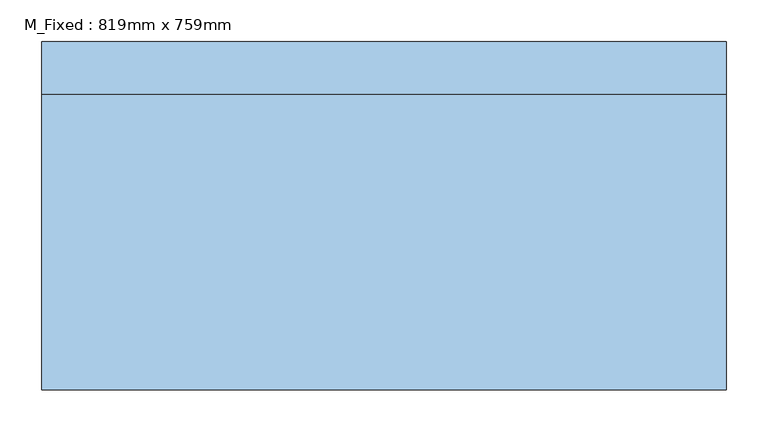
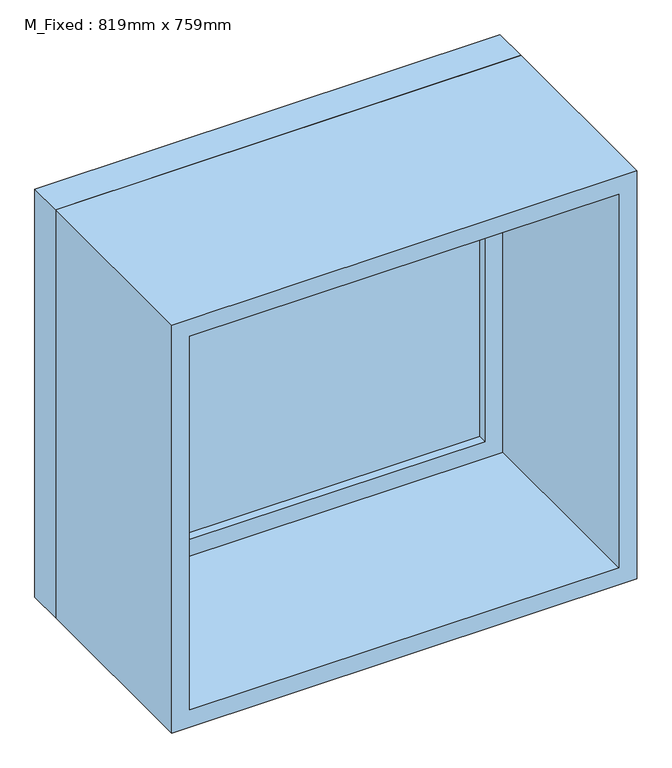
"""IFC4 building model written with IfcOpenShell, lengths in millimetres: window geometry, M_Fixed : 819mm x 759mm."""

from ifc_helpers import new_model, si_unit, frame, origin, place, context, project, spatial, polyline, outline, extrude, source, transform, mapped, element, save


def m_fixed_819mm_x_759mm_7938e442(model_context):
    return source(origin(), model_context, "Body", "SweptSolid", [
        extrude(outline(polyline([(-346.5, 186.5), (346.5, 186.5), (346.5, 174.5), (-346.5, 174.5), (-346.5, 186.5)])), frame((0.0, 0.0, 163.0), z_axis=(0.0, 0.0, 1.0), x_axis=(1.0, 0.0, 0.0)), (0.0, 0.0, 1.0), 633.0),
        extrude(outline(polyline([(840.0, -390.5), (119.0, -390.5), (119.0, 390.5), (840.0, 390.5), (840.0, -390.5)]), holes=[polyline([(796.0, -346.5), (796.0, 346.5), (163.0, 346.5), (163.0, -346.5), (796.0, -346.5)])]), frame((0.0, 158.5, 0.0), z_axis=(0.0, 1.0, 0.0), x_axis=(0.0, 0.0, 1.0)), (0.0, 0.0, 1.0), 44.0),
        extrude(outline(polyline([(859.0, -409.5), (100.0, -409.5), (100.0, 409.5), (859.0, 409.5), (859.0, -409.5)]), holes=[polyline([(840.0, -390.5), (840.0, 390.5), (119.0, 390.5), (119.0, -390.5), (840.0, -390.5)])]), frame((0.0, 158.5, 0.0), z_axis=(0.0, 1.0, 0.0), x_axis=(0.0, 0.0, 1.0)), (0.0, 0.0, 1.0), 63.0),
        extrude(outline(polyline([(859.0, -409.5), (100.0, -409.5), (100.0, 409.5), (859.0, 409.5), (859.0, -409.5)]), holes=[polyline([(827.0, -377.5), (827.0, 377.5), (132.0, 377.5), (132.0, -377.5), (827.0, -377.5)])]), frame((0.0, -195.5, 0.0), z_axis=(0.0, 1.0, 0.0), x_axis=(0.0, 0.0, 1.0)), (0.0, 0.0, 1.0), 354.0),
    ])


if __name__ == "__main__":
    model = new_model("IFC4")
    model_context = context("Model", 3, world=origin())
    ifc_project = project(units=[si_unit("LENGTHUNIT", "METRE", prefix="MILLI")], contexts=[model_context])
    site = spatial("IfcSite", under=ifc_project)
    building = spatial("IfcBuilding", under=site)
    placement = place(None, origin())
    m_fixed_819mm_x_759mm_shape = m_fixed_819mm_x_759mm_7938e442(model_context)
    element("IfcWindow", 1, ObjectType="M_Fixed : 819mm x 759mm", at=placement, inside=building, context=model_context, shape_type="MappedRepresentation", body=[
        mapped(m_fixed_819mm_x_759mm_shape, transform((0.0, 0.0, 0.0), x_axis=(1.0, 0.0, 0.0), y_axis=(0.0, 1.0, 0.0), z_axis=(0.0, 0.0, 1.0))),
    ])
    save(model, "model.ifc")

# Revit data of these elements
# Type "M_Fixed : 819mm x 759mm"
#   Manufacturer = "Manufacturer"
#   Type Mark = "02"
#   Construction Type = "Construction Type"
#   AccessibilityPerformance = "AccessibilityPerformance"
#   CodePerformance = "CodePerformance"
#   ConfigurationType = "ConfigurationType"
#   ConstructionType = "ConstructionType"
#   FireRating = "FireRating"
#   GlazingAreaFraction = "GlazingAreaFraction"
#   OperationType = "OperationType"
#   Area = "Area"
#   Color = "Color"
#   Constituents = "Constituents"
#   Features = "Features"
#   Finish = "Finish"
#   Grade = "Grade"
#   Material = "Material"
#   ModelReference = "ModelReference"
#   NominalHeight = "NominalHeight"
#   NominalLength = "NominalLength"
#   NominalWidth = "NominalWidth"
#   ProductionYear = "ProductionYear"
#   Reference = "Reference"
#   Shape = "Shape"
#   Size = "Size"
#   SustainabilityPerformance = "SustainabilityPerformance"
#   WarrantyDescription = "WarrantyDescription"
#   WarrantyDurationLabor = "WarrantyDurationLabor"
#   WarrantyDurationParts = "WarrantyDurationParts"
#   WarrantyGuarantorLabor = "WarrantyGuarantorLabor"
#   WarrantyGuarantorParts = "WarrantyGuarantorParts"
#   ExpectedLife = "ExpectedLife"
#   ReplacementCost = "ReplacementCost"
#   AssetAccountingType = "FIXED"
#   ModelLabel = "ModelLabel"
#   Height = 0.759 m
#   Default Sill Height = 0.100 m
#   Width = 0.819 m
#   Window Inset = 0.019 m
#   Frame Exterior Material = Sash
#   Frame Interior Material = Sash
#   Glass Pane Material = Glass
#   Sash = Sash
#   Wall Closure = (empty or 0)
# Element 1 (IfcWindow, "M_Fixed : 819mm x 759mm")
#   Materials on its faces: "Sash", "Glass"
# Materials
#   "Sash": class "Wood", colour RGB 224 178 126, transparency 0
#   "Glass": class "Glass", colour RGB 0 128 192, transparency 0.9
